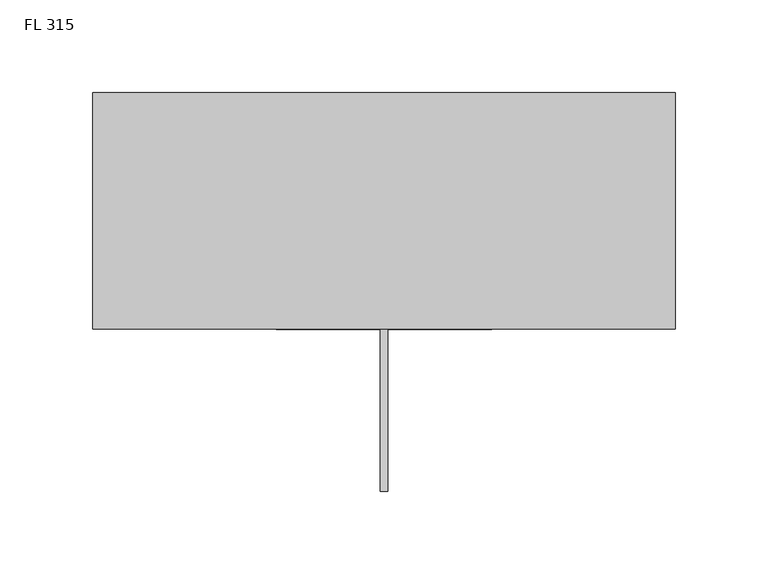
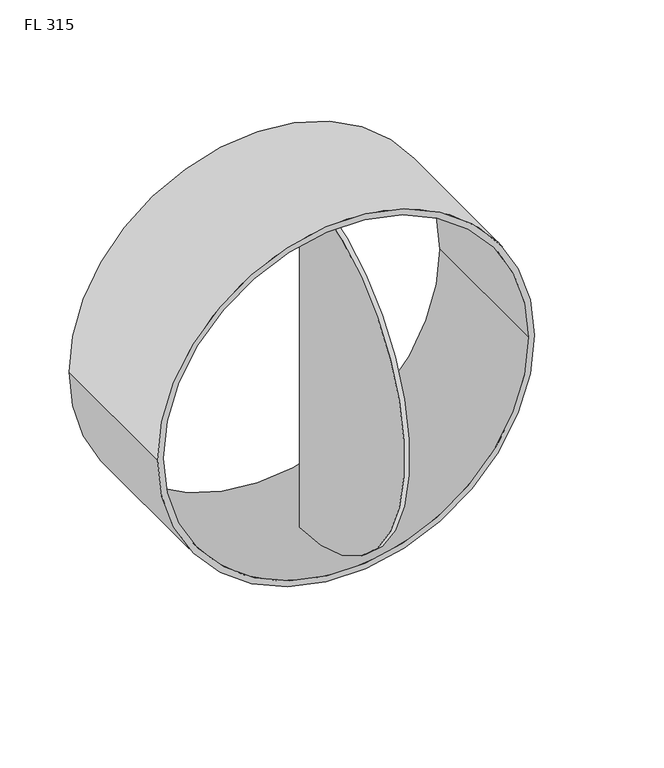
"""IFC4 building model written with IfcOpenShell, lengths in millimetres: proxy geometry, Обратный клапан круглый FL : FL 315."""

from ifc_helpers import new_model, si_unit, point, frame, origin, origin_2d, place, context, project, spatial, polyline, circle_curve, trimmed, segment, composite_curve, outline, extrude, source, transform, mapped, element, save


def fl_315_e08b723a(model_context):
    return source(origin(), model_context, "Body", "SweptSolid", [
        extrude(outline(composite_curve([segment(trimmed(circle_curve(origin_2d(), 152.5), [point((0.0, -152.5))], [point((0.0, 152.5))], False, "CARTESIAN"), True, "CONTINUOUS"), segment(polyline([(0.0, 152.5), (0.0, -152.5)]), True, "CONTINUOUS")], self_intersect=False)), frame((-2.0, 0.0, 0.0), z_axis=(1.0, 0.0, 0.0), x_axis=(0.0, 1.0, 0.0)), (0.0, 0.0, 1.0), 4.0),
        extrude(outline(composite_curve([segment(trimmed(circle_curve(origin_2d(), 157.5), [point((0.0, -157.5))], [point((0.0, 157.5))], False, "CARTESIAN"), True, "CONTINUOUS"), segment(trimmed(circle_curve(origin_2d(), 157.5), [point((0.0, 157.5))], [point((0.0, -157.5))], False, "CARTESIAN"), True, "CONTINUOUS")], self_intersect=False), holes=[composite_curve([segment(trimmed(circle_curve(origin_2d(), 152.5), [point((0.0, -152.5))], [point((0.0, 152.5))], True, "CARTESIAN"), True, "CONTINUOUS"), segment(trimmed(circle_curve(origin_2d(), 152.5), [point((0.0, 152.5))], [point((0.0, -152.5))], True, "CARTESIAN"), True, "CONTINUOUS")], self_intersect=False)]), frame((0.0, -64.0, 0.0), z_axis=(0.0, 1.0, 0.0), x_axis=(0.0, 0.0, 1.0)), (0.0, 0.0, 1.0), 128.0),
    ])


if __name__ == "__main__":
    model = new_model("IFC4")
    model_context = context("Model", 3, world=origin())
    ifc_project = project(units=[si_unit("LENGTHUNIT", "METRE", prefix="MILLI")], contexts=[model_context])
    site = spatial("IfcSite", under=ifc_project)
    building = spatial("IfcBuilding", under=site)
    placement = place(None, origin())
    fl_315_shape = fl_315_e08b723a(model_context)
    element("IfcBuildingElementProxy", 1, Name="Обратный клапан круглый FL : FL 315", ObjectType="Обратный клапан круглый FL : FL 315", at=placement, inside=building, context=model_context, shape_type="MappedRepresentation", body=[
        mapped(fl_315_shape, transform((0.0, 0.0, 0.0), x_axis=(1.0, 0.0, 0.0), y_axis=(0.0, 1.0, 0.0), z_axis=(0.0, 0.0, 1.0))),
    ])
    save(model, "model.ifc")

# Revit data of these elements
# Type "Обратный клапан круглый FL : FL 315"
#   ADSK_Система_Имя [instance default] = ""
#   ADSK_Наименование краткое = "FL 315"
#   ADSK_Наименование [instance default] = "Обратный клапан FL 315"
#   ADSK_Масса_Текст = "0.81"
#   ADSK_Марка = ""
#   ADSK_Код изделия = ""
#   ADSK_Завод-изготовитель = "WAER"
#   ADSK_Единица измерения = "шт."
#   ADSK_URL страницы изделия = ""
#   ADSK_URL документации изделия = ""
#   ADSK_Расход воздуха = 0 m³/h
#   ADSK_Размер_Длина_L = 128 mm
#   ADSK_Размер_Диаметр_D1 = 305 mm
#   ADSK_Размер_Диаметр_D = 315 mm
#   ADSK_Потеря давления воздуха = 0.0 Pa
#   ADSK_Масса = 0.81
#   ADSK_Количество [instance default] = 1
#   Default Elevation = 0
#   URL = ""
#   Cost = 0
